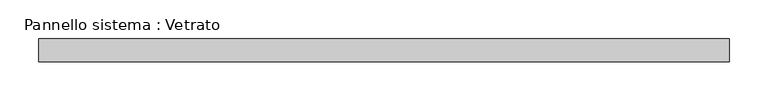
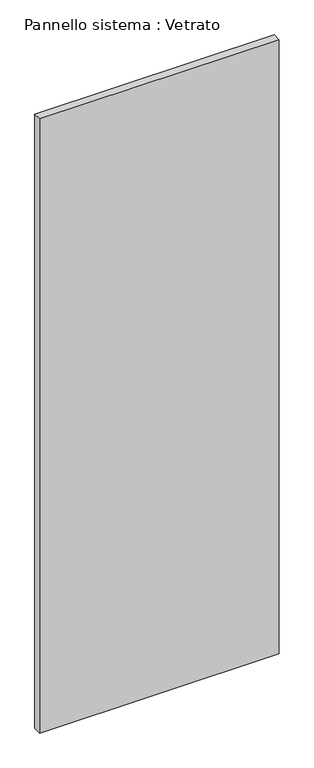
"""IFC4 building model written with IfcOpenShell, lengths in millimetres: plate geometry, Pannello sistema : Vetrato."""

import ifcopenshell
import ifcopenshell.guid

model = None  # the IFC model being written
_history = None  # IfcOwnerHistory: only IFC2X3 demands one
_inside = {}  # id of a spatial element -> (the spatial element, [elements in it])
_under = {}  # id of a project, library or spatial element -> (it, [spatial elements below it])
_declared = {}  # id of a project -> (the project, [libraries it declares])
_typed = {}  # id of a type object -> (the type object, [elements of that type])
_made_of = {}  # id of a material, layer set ... -> (it, [elements and type objects made of it])


def new_model(schema):
    """Start an empty IFC model of exactly this schema.

    Asked for "IFC4X3", IfcOpenShell would pick the latest addendum, in which some entities
    have other attributes; the version numbers below select the first issue.
    IFC2X3 requires an IfcOwnerHistory on every rooted entity: one is made here for all.
    """
    global model, _history
    if schema == "IFC4X3":
        model = ifcopenshell.file(schema_version=(4, 3, 0, 0))
    else:
        model = ifcopenshell.file(schema=schema)
    _inside.clear()
    _under.clear()
    _declared.clear()
    _typed.clear()
    _made_of.clear()
    _history = None
    if model.schema == "IFC2X3":
        org = make("IfcOrganization", Name="unknown")
        user = make(
            "IfcPersonAndOrganization",
            ThePerson=make("IfcPerson", FamilyName="unknown"),
            TheOrganization=org,
        )
        app = make(
            "IfcApplication",
            ApplicationDeveloper=org,
            Version="unknown",
            ApplicationFullName="unknown",
            ApplicationIdentifier="unknown",
        )
        _history = make(
            "IfcOwnerHistory",
            OwningUser=user,
            OwningApplication=app,
            ChangeAction="ADDED",
            CreationDate=0,
        )
    return model


def make(cls, **values):
    """One entity of the class cls with the attributes given. An attribute that is None is left unset."""
    return model.create_entity(
        cls, **{name: value for name, value in values.items() if value is not None}
    )


def rooted(cls, **values):
    """An entity with a GlobalId (a new one), such as an element, a storey or a relation."""
    return make(cls, GlobalId=ifcopenshell.guid.new(), OwnerHistory=_history, **values)


def si_unit(unit_type, name, prefix=None):
    """IfcSIUnit, for example si_unit("LENGTHUNIT", "METRE", prefix="MILLI")."""
    return make("IfcSIUnit", UnitType=unit_type, Prefix=prefix, Name=name)


def assignment(units):
    """IfcUnitAssignment: the units of a project."""
    return None if units is None else make("IfcUnitAssignment", Units=units)


def point(xyz):
    """IfcCartesianPoint."""
    return None if xyz is None else make("IfcCartesianPoint", Coordinates=xyz)


def direction(xyz):
    """IfcDirection."""
    return None if xyz is None else make("IfcDirection", DirectionRatios=xyz)


def frame(location, z_axis=None, x_axis=None):
    """IfcAxis2Placement3D, a coordinate frame: its origin and axes. An axis left out is left unset."""
    return make(
        "IfcAxis2Placement3D",
        Location=point(location),
        Axis=direction(z_axis),
        RefDirection=direction(x_axis),
    )


def origin():
    """The frame at (0, 0, 0) with its axes left unset."""
    return frame((0.0, 0.0, 0.0))


def origin_with_axes():
    """The frame at (0, 0, 0) with the z axis (0, 0, 1) and the x axis (1, 0, 0) written out."""
    return frame((0.0, 0.0, 0.0), z_axis=(0.0, 0.0, 1.0), x_axis=(1.0, 0.0, 0.0))


def place(relative_to, where):
    """IfcLocalPlacement: puts the frame where relative to a parent placement (None: the world)."""
    return make(
        "IfcLocalPlacement", PlacementRelTo=relative_to, RelativePlacement=where
    )


def context(
    kind, dimensions, precision=None, world=None, true_north=None, identifier=None
):
    """IfcGeometricRepresentationContext, for example the 3D "Model" context."""
    return make(
        "IfcGeometricRepresentationContext",
        ContextIdentifier=identifier,
        ContextType=kind,
        CoordinateSpaceDimension=dimensions,
        Precision=precision,
        WorldCoordinateSystem=world,
        TrueNorth=true_north,
    )


def project(units=None, contexts=None):
    """IfcProject with its units and contexts."""
    return rooted(
        "IfcProject",
        Name="project",
        RepresentationContexts=contexts,
        UnitsInContext=assignment(units),
    )


def spatial(cls, under=None, at=None, **own):
    """A site, building, storey or space (cls), placed at a placement, below another one or the project."""
    s = rooted(cls, ObjectPlacement=at, **own)
    if under is not None:
        _under.setdefault(under.id(), (under, []))[1].append(s)
    return s


def polyline(points):
    """IfcPolyline through the points."""
    return make("IfcPolyline", Points=[point(p) for p in points])


def outline(outer, holes=None, kind="AREA"):
    """IfcArbitraryClosedProfileDef: a profile drawn as a closed curve; with holes, ...WithVoids."""
    if holes is None:
        return make("IfcArbitraryClosedProfileDef", ProfileType=kind, OuterCurve=outer)
    return make(
        "IfcArbitraryProfileDefWithVoids",
        ProfileType=kind,
        OuterCurve=outer,
        InnerCurves=holes,
    )


def extrude(swept, where, along, depth):
    """IfcExtrudedAreaSolid: the profile swept, set in the frame where, extruded along a direction by depth."""
    return make(
        "IfcExtrudedAreaSolid",
        SweptArea=swept,
        Position=where,
        ExtrudedDirection=direction(along),
        Depth=depth,
    )


def shape(context_of_items, identifier, shape_type, items):
    """IfcShapeRepresentation: the items that make up one representation, for example the "Body"."""
    return make(
        "IfcShapeRepresentation",
        ContextOfItems=context_of_items,
        RepresentationIdentifier=identifier,
        RepresentationType=shape_type,
        Items=items,
    )


def source(mapping_origin, context_of_items, identifier, shape_type, items):
    """IfcRepresentationMap: a shape defined once, which mapped items show again and again."""
    return make(
        "IfcRepresentationMap",
        MappingOrigin=mapping_origin,
        MappedRepresentation=shape(context_of_items, identifier, shape_type, items),
    )


def transform(
    local_origin,
    x_axis=None,
    y_axis=None,
    z_axis=None,
    scale=None,
    scale2=None,
    scale3=None,
    uniform=True,
):
    """IfcCartesianTransformationOperator3D, or its non-uniform kind. x_axis, y_axis, z_axis: its Axis1, 2, 3."""
    if uniform:
        return make(
            "IfcCartesianTransformationOperator3D",
            Axis1=direction(x_axis),
            Axis2=direction(y_axis),
            LocalOrigin=point(local_origin),
            Scale=scale,
            Axis3=direction(z_axis),
        )
    return make(
        "IfcCartesianTransformationOperator3DnonUniform",
        Axis1=direction(x_axis),
        Axis2=direction(y_axis),
        LocalOrigin=point(local_origin),
        Scale=scale,
        Axis3=direction(z_axis),
        Scale2=scale2,
        Scale3=scale3,
    )


def mapped(mapping_source, mapping_target):
    """IfcMappedItem: shows the shape of a source again, moved by a transform."""
    return make(
        "IfcMappedItem", MappingSource=mapping_source, MappingTarget=mapping_target
    )


def made_of(thing, what):
    """Note that an element or type object is made of a material, layer set ...; save() writes the relation."""
    if what is not None:
        _made_of.setdefault(what.id(), (what, []))[1].append(thing)
    return thing


def element(
    cls,
    number,
    at=None,
    inside=None,
    cuts=None,
    type_object=None,
    material=None,
    context=None,
    identifier="Body",
    shape_type=None,
    held_by="IfcProductDefinitionShape",
    body=None,
    shapes=None,
    **own,
):
    """One element of the class cls, such as IfcWall. Its Tag is "e" and its number.

    at: its placement. inside: the storey or other place that contains it. cuts: it is an
    opening in that element (IfcRelVoidsElement). A single representation is given by context,
    identifier, shape_type and body (its items); several are given by shapes. held_by: the class
    of the entity that holds the representations. save() writes the other relations.
    """
    e = rooted(cls, Tag="e%d" % number, ObjectPlacement=at, **own)
    if body is not None:
        shapes = [shape(context, identifier, shape_type, body)]
    if shapes is not None:
        e.Representation = make(held_by, Representations=shapes)
    if inside is not None:
        _inside.setdefault(inside.id(), (inside, []))[1].append(e)
    if cuts is not None:
        rooted(
            "IfcRelVoidsElement", RelatingBuildingElement=cuts, RelatedOpeningElement=e
        )
    if type_object is not None:
        _typed.setdefault(type_object.id(), (type_object, []))[1].append(e)
    return made_of(e, material)


def aggregate(whole, parts):
    """IfcRelAggregates: a whole, such as a stair, and the parts it consists of."""
    return rooted("IfcRelAggregates", RelatingObject=whole, RelatedObjects=parts)


def save(model, path):
    """Write the relations noted so far, then the file.

    IfcRelAggregates (storeys below a building ...), IfcRelContainedInSpatialStructure (elements
    in a storey), IfcRelDefinesByType, IfcRelAssociatesMaterial and IfcRelDeclares: one each for
    every whole, place, type object, material and project.
    """
    for whole, parts in _under.values():
        aggregate(whole, parts)
    for where, things in _inside.values():
        rooted(
            "IfcRelContainedInSpatialStructure",
            RelatedElements=things,
            RelatingStructure=where,
        )
    for kind, things in _typed.values():
        rooted("IfcRelDefinesByType", RelatedObjects=things, RelatingType=kind)
    for what, things in _made_of.values():
        rooted("IfcRelAssociatesMaterial", RelatedObjects=things, RelatingMaterial=what)
    for by, libraries in _declared.values():
        rooted("IfcRelDeclares", RelatingContext=by, RelatedDefinitions=libraries)
    model.write(path)


def pannello_sistema_vetrato_1d2d4d6f(model_context):
    return source(origin(), model_context, "Body", "SweptSolid", [
        extrude(outline(polyline([(447.5, -15.0), (-447.5, -15.0), (-447.5, 15.0), (447.5, 15.0), (447.5, -15.0)])), origin_with_axes(), (0.0, 0.0, 1.0), 2425.0),
    ])


if __name__ == "__main__":
    model = new_model("IFC4")
    model_context = context("Model", 3, world=origin())
    ifc_project = project(units=[si_unit("LENGTHUNIT", "METRE", prefix="MILLI")], contexts=[model_context])
    site = spatial("IfcSite", under=ifc_project)
    building = spatial("IfcBuilding", under=site)
    placement = place(None, origin())
    pannello_sistema_vetrato_shape = pannello_sistema_vetrato_1d2d4d6f(model_context)
    element("IfcPlate", 1, ObjectType="Pannello sistema : Vetrato", at=placement, inside=building, context=model_context, shape_type="MappedRepresentation", body=[
        mapped(pannello_sistema_vetrato_shape, transform((0.0, 0.0, 0.0), x_axis=(1.0, 0.0, 0.0), y_axis=(0.0, 1.0, 0.0), z_axis=(0.0, 0.0, 1.0))),
    ])
    save(model, "model.ifc")

# Revit data of these elements
# Type "Pannello sistema : Vetrato"
#   Construction Type Id = "GSP4R"
#   Analytic Construction = "Vetrata singola Pilkington 1/8 in"
#   Visual Light Transmittance = 0.9
#   Solar Heat Gain Coefficient = 0.86
#   Heat Transfer Coefficient (U) = 6.7069 W/(m²·K)
# Element 1 (IfcPlate, "Pannello sistema : Vetrato")
#   Materials on its faces: "Default - Vetro"
# Materials
#   "Default - Vetro": class "Vetro", colour RGB 208 208 208, transparency 0.7, Cost = 0
